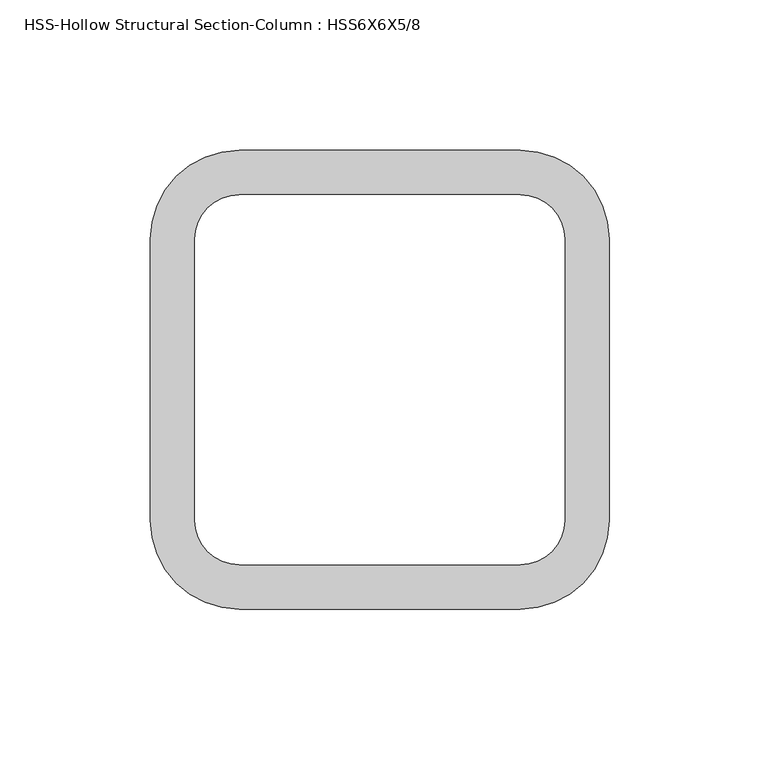
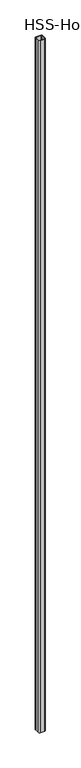
"""IFC4 building model written with IfcOpenShell, lengths in millimetres: column geometry, HSS-Hollow Structural Section-Column : HSS6X6X5/8."""

from ifc_helpers import new_model, si_unit, point, frame, frame_2d, origin, place, context, project, spatial, polyline, circle_curve, trimmed, segment, composite_curve, outline, extrude, source, transform, mapped, element, save


def hss_hollow_structural_section_column_hss6x6x5_8_d9445e73(model_context):
    return source(origin(), model_context, "Body", "SweptSolid", [
        extrude(outline(composite_curve([segment(trimmed(circle_curve(frame_2d((46.6852, 46.6852)), 29.5148), [point((46.6852, 76.2))], [point((76.2, 46.6852))], False, "CARTESIAN"), True, "CONTINUOUS"), segment(polyline([(76.2, 46.6852), (76.2, -46.6852)]), True, "CONTINUOUS"), segment(trimmed(circle_curve(frame_2d((46.6852, -46.6852)), 29.5148), [point((76.2, -46.6852))], [point((46.6852, -76.2))], False, "CARTESIAN"), True, "CONTINUOUS"), segment(polyline([(46.6852, -76.2), (-46.6852, -76.2)]), True, "CONTINUOUS"), segment(trimmed(circle_curve(frame_2d((-46.6852, -46.6852)), 29.5148), [point((-46.6852, -76.2))], [point((-76.2, -46.6852))], False, "CARTESIAN"), True, "CONTINUOUS"), segment(polyline([(-76.2, -46.6852), (-76.2, 46.6852)]), True, "CONTINUOUS"), segment(trimmed(circle_curve(frame_2d((-46.6852, 46.6852)), 29.5148), [point((-76.2, 46.6852))], [point((-46.6852, 76.2))], False, "CARTESIAN"), True, "CONTINUOUS"), segment(polyline([(-46.6852, 76.2), (46.6852, 76.2)]), True, "CONTINUOUS")], self_intersect=False), holes=[composite_curve([segment(polyline([(46.6852, 61.4426), (-46.6852, 61.4426)]), True, "CONTINUOUS"), segment(trimmed(circle_curve(frame_2d((-46.6852, 46.6852)), 14.7574), [point((-46.6852, 61.4426))], [point((-61.4426, 46.6852))], True, "CARTESIAN"), True, "CONTINUOUS"), segment(polyline([(-61.4426, 46.6852), (-61.4426, -46.6852)]), True, "CONTINUOUS"), segment(trimmed(circle_curve(frame_2d((-46.6852, -46.6852)), 14.7574), [point((-61.4426, -46.6852))], [point((-46.6852, -61.4426))], True, "CARTESIAN"), True, "CONTINUOUS"), segment(polyline([(-46.6852, -61.4426), (46.6852, -61.4426)]), True, "CONTINUOUS"), segment(trimmed(circle_curve(frame_2d((46.6852, -46.6852)), 14.7574), [point((46.6852, -61.4426))], [point((61.4426, -46.6852))], True, "CARTESIAN"), True, "CONTINUOUS"), segment(polyline([(61.4426, -46.6852), (61.4426, 46.6852)]), True, "CONTINUOUS"), segment(trimmed(circle_curve(frame_2d((46.6852, 46.6852)), 14.7574), [point((61.4426, 46.6852))], [point((46.6852, 61.4426))], True, "CARTESIAN"), True, "CONTINUOUS")], self_intersect=False)]), frame((0.0, 0.0, -3657.6), z_axis=(0.0, 0.0, 1.0), x_axis=(1.0, 0.0, 0.0)), (0.0, 0.0, 1.0), 15925.8),
    ])


if __name__ == "__main__":
    model = new_model("IFC4")
    model_context = context("Model", 3, world=origin())
    ifc_project = project(units=[si_unit("LENGTHUNIT", "METRE", prefix="MILLI")], contexts=[model_context])
    site = spatial("IfcSite", under=ifc_project)
    building = spatial("IfcBuilding", under=site)
    placement = place(None, origin())
    hss_hollow_structural_section_column_hss6x6x5_8_shape = hss_hollow_structural_section_column_hss6x6x5_8_d9445e73(model_context)
    element("IfcColumn", 1, ObjectType="HSS-Hollow Structural Section-Column : HSS6X6X5/8", at=placement, inside=building, context=model_context, shape_type="MappedRepresentation", body=[
        mapped(hss_hollow_structural_section_column_hss6x6x5_8_shape, transform((0.0, 0.0, 0.0), x_axis=(1.0, 0.0, 0.0), y_axis=(0.0, 1.0, 0.0), z_axis=(0.0, 0.0, 1.0))),
    ])
    save(model, "model.ifc")

# Revit data of these elements
# Type "HSS-Hollow Structural Section-Column : HSS6X6X5/8"
#   Assembly Code = "B10"
#   Shape = "Square"
#   W = 42.1
#   Ht = 0' - 6"
#   b = 0' - 6"
#   kr = 0' - 1.162"
#   t = 0' - 0.581"
#   A = 0.08125 SF
#   Structural Material [instance default] = Steel ASTM A500, Grade B, Rectangular and Square
# Element 1 (IfcColumn, "HSS-Hollow Structural Section-Column : HSS6X6X5/8")
#   Materials on its faces: "Steel ASTM A500, Grade B, Rectangular and Square"
# Materials
#   "Steel ASTM A500, Grade B, Rectangular and Square": class "Metal", colour RGB 199 199 199, transparency 0, Description = "Carbon steel", Cost = 0
